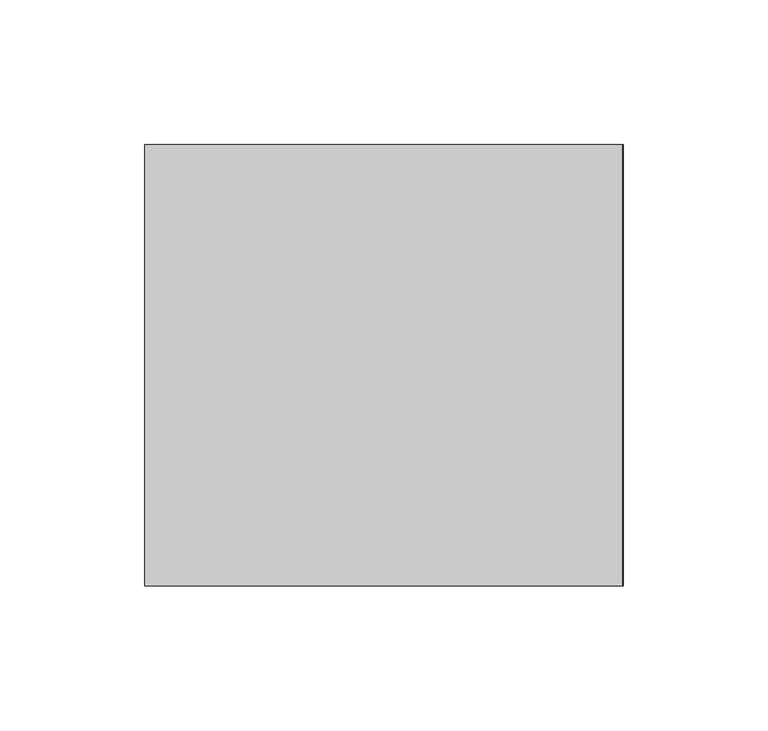
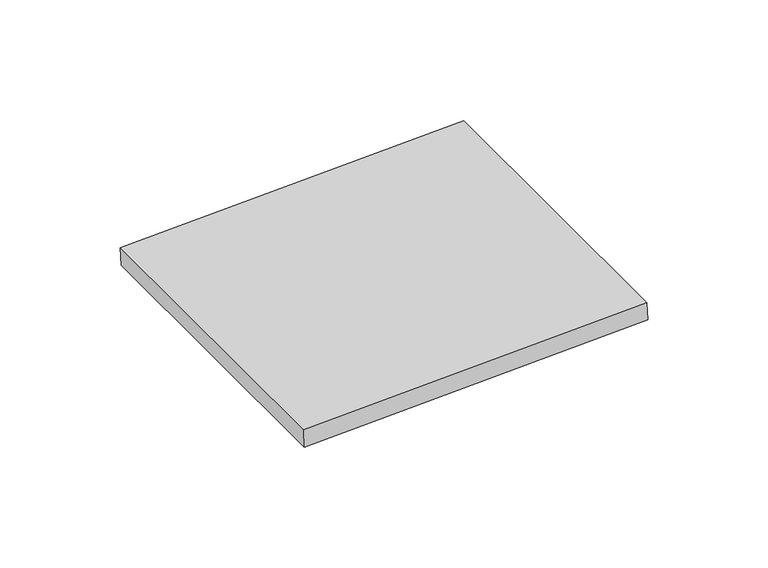
"""IFC4 building model written with IfcOpenShell, lengths in millimetres: proxy geometry, Generic Models 7:Generic Models 1:8:Generic Models 1:8 : Generic Models 7:Generic Models 1:337419:48 : Generic Models 7:Generic Models 1:8:Generic Models 1:8 : Generic Models 7:Generic Models 1:337419:315935."""

from ifc_helpers import new_model, si_unit, frame, origin, place, context, project, spatial, polyline, outline, extrude, source, transform, mapped, element, save


def generic_models_656a813f(model_context):
    return source(origin(), model_context, "Body", "SweptSolid", [
        extrude(outline(polyline([(0.0, -164.8422109), (0.0, 0.0), (152.4, 0.0), (152.4, -164.8422109), (0.0, -164.8422109)])), frame((560759.5235326, -578260.4833448, 3696.8191169), z_axis=(-0.04163054483311677, 0.0, 0.999133073087313), x_axis=(0.0, -1.0, 0.0)), (0.0, 0.0, 1.0), 8.89),
    ])


if __name__ == "__main__":
    model = new_model("IFC4")
    model_context = context("Model", 3, world=origin())
    ifc_project = project(units=[si_unit("LENGTHUNIT", "METRE", prefix="MILLI")], contexts=[model_context])
    site = spatial("IfcSite", under=ifc_project)
    building = spatial("IfcBuilding", under=site)
    placement = place(None, origin())
    generic_models_shape = generic_models_656a813f(model_context)
    element("IfcBuildingElementProxy", 1, Name="Generic Models 7:Generic Models 1:8:Generic Models 1:8 : Generic Models 7:Generic Models 1:337419:48 : Generic Models 7:Generic Models 1:8:Generic Models 1:8 : Generic Models 7:Generic Models 1:337419:315935", ObjectType="Generic Models 7:Generic Models 1:8:Generic Models 1:8 : Generic Models 7:Generic Models 1:337419:48 : Generic Models 7:Generic Models 1:8:Generic Models 1:8 : Generic Models 7:Generic Models 1:337419:315935", at=placement, inside=building, context=model_context, shape_type="MappedRepresentation", body=[
        mapped(generic_models_shape, transform((0.0, 0.0, 0.0), x_axis=(1.0, 0.0, 0.0), y_axis=(0.0, 1.0, 0.0), z_axis=(0.0, 0.0, 1.0))),
    ])
    save(model, "model.ifc")

# Revit data of these elements
# Type "Generic Models 7:Generic Models 1:8:Generic Models 1:8 : Generic Models 7:Generic Models 1:337419:48 : Generic Models 7:Generic Models 1:8:Generic Models 1:8 : Generic Models 7:Generic Models 1:337419:315935"
#   NameOverride = "Generic Models 7:Generic Models 1:8:Generic Models 1:8 : Generic Models 7:Generic Models 1:337419:315935"
#   ObjectTypeOverride = "Generic Models 1:8 : Generic Models 7:Generic Models 1:337419"
#   Reference = "Generic Models 1"
#   Tag = "315935"
# Element 1 (IfcBuildingElementProxy, "Generic Models 7:Generic Models 1:8:Generic Models 1:8 : Generic Models 7:Generic Models 1:337419:48 : Generic Models 7:Generic Models 1:8:Generic Models 1:8 : Generic Models 7:Generic Models 1:337419:315935")
#   Materials on its faces: "STRUCTURAL STEEL - SEE STRUCT. DWGS"
# Materials
#   "STRUCTURAL STEEL - SEE STRUCT. DWGS": class "Metal", colour RGB 189 187 185, transparency 0, Description = "Structural steel 50ksi", Cost = 0
